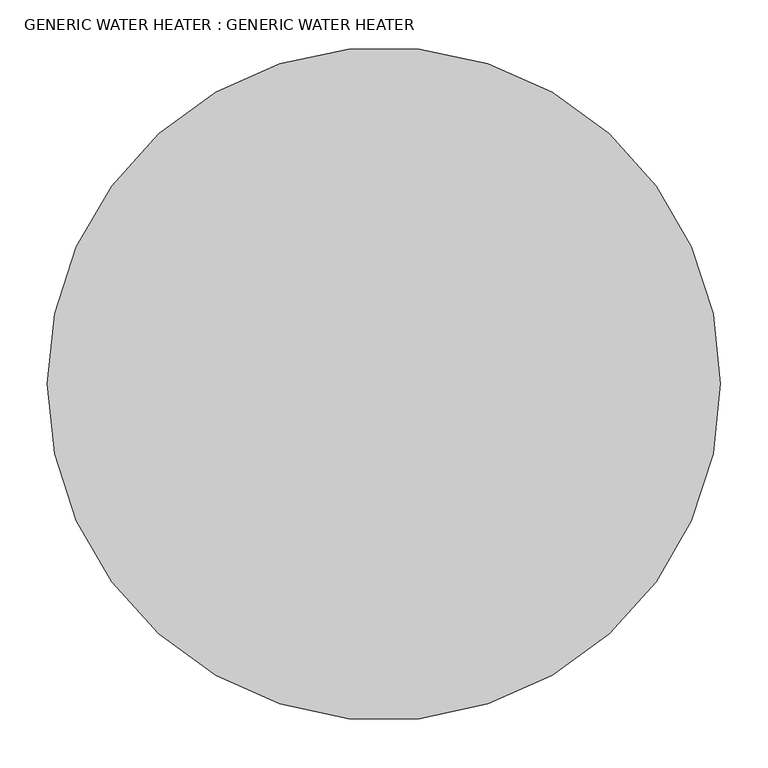
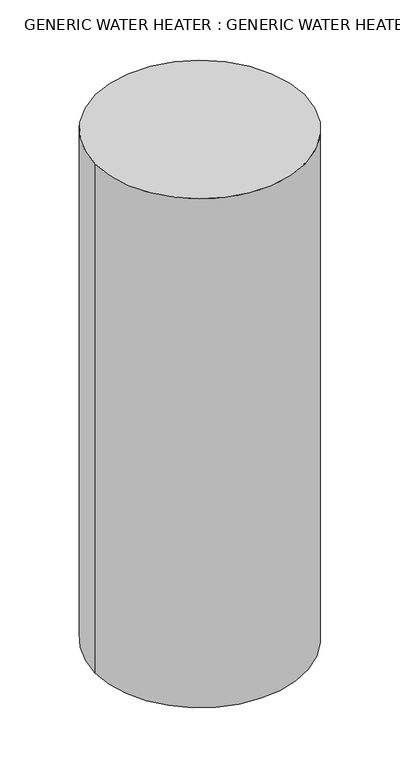
"""IFC4 building model written with IfcOpenShell, lengths in millimetres: proxy geometry, GENERIC WATER HEATER : GENERIC WATER HEATER."""

from ifc_helpers import new_model, si_unit, point, origin, origin_with_axes, origin_2d, place, context, project, spatial, circle_curve, trimmed, segment, composite_curve, outline, extrude, source, transform, mapped, element, save


def generic_water_heater_generic_water_heater_aa4aec31(model_context):
    return source(origin(), model_context, "Body", "SweptSolid", [
        extrude(outline(composite_curve([segment(trimmed(circle_curve(origin_2d(), 355.6), [point((-355.6, 0.0))], [point((355.6, 0.0))], False, "CARTESIAN"), True, "CONTINUOUS"), segment(trimmed(circle_curve(origin_2d(), 355.6), [point((355.6, 0.0))], [point((-355.6, 0.0))], False, "CARTESIAN"), True, "CONTINUOUS")], self_intersect=False)), origin_with_axes(), (0.0, 0.0, 1.0), 1828.8),
    ])


if __name__ == "__main__":
    model = new_model("IFC4")
    model_context = context("Model", 3, world=origin())
    ifc_project = project(units=[si_unit("LENGTHUNIT", "METRE", prefix="MILLI")], contexts=[model_context])
    site = spatial("IfcSite", under=ifc_project)
    building = spatial("IfcBuilding", under=site)
    placement = place(None, origin())
    generic_water_heater_generic_water_heater_shape = generic_water_heater_generic_water_heater_aa4aec31(model_context)
    element("IfcBuildingElementProxy", 1, Name="GENERIC WATER HEATER : GENERIC WATER HEATER", ObjectType="GENERIC WATER HEATER : GENERIC WATER HEATER", at=placement, inside=building, context=model_context, shape_type="MappedRepresentation", body=[
        mapped(generic_water_heater_generic_water_heater_shape, transform((0.0, 0.0, 0.0), x_axis=(1.0, 0.0, 0.0), y_axis=(0.0, 1.0, 0.0), z_axis=(0.0, 0.0, 1.0))),
    ])
    save(model, "model.ifc")
